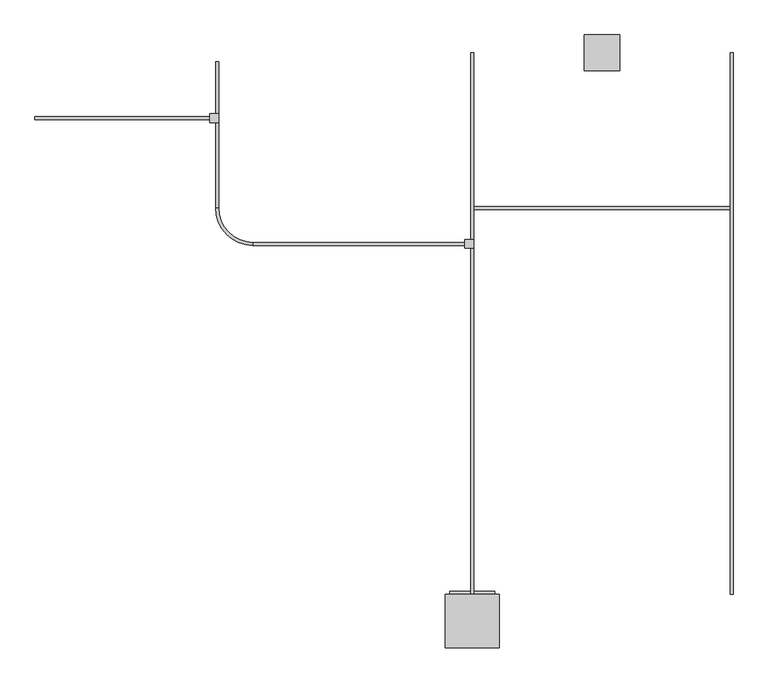
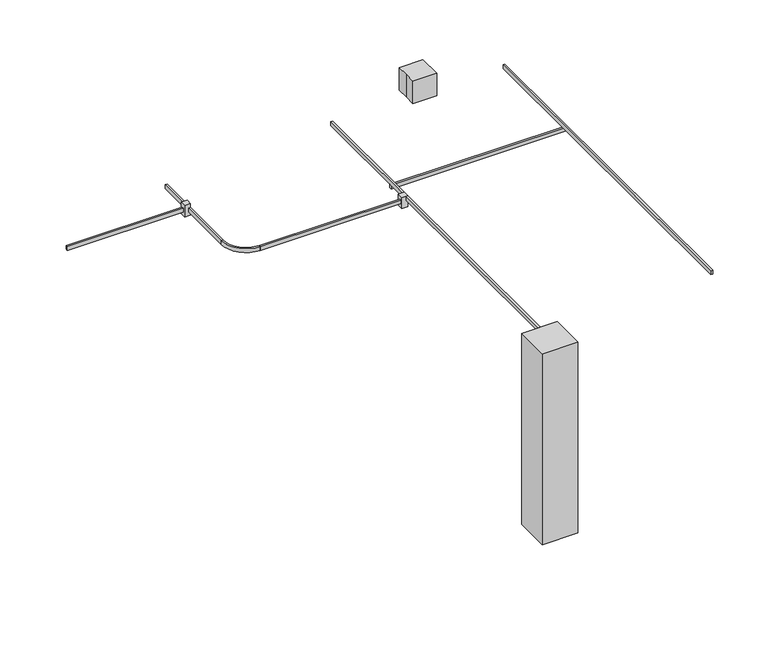
"""IFC4 building model written with IfcOpenShell, lengths in millimetres: proxy geometry, A1205 - Lift System, Overhead, Patient Room w-Bath-mirror : A1205 - Lift System, Overhead, Patient Room w-Bath-mirror."""

from ifc_helpers import new_model, si_unit, point, frame, frame_2d, origin, origin_with_axes, place, context, project, spatial, polyline, circle_curve, trimmed, segment, composite_curve, outline, extrude, source, transform, mapped, element, save


def specialty_equipment_7046e059(model_context):
    return source(origin(), model_context, "Body", "SweptSolid", [
        extrude(outline(polyline([(-3338.4200386, -545.1376019), (-3338.4200386, -570.5376019), (-4825.7229408, -570.5376019), (-4825.7229408, -545.1376019), (-3338.4200386, -545.1376019)])), frame((0.0, 0.0, -101.6), z_axis=(0.0, 0.0, 1.0), x_axis=(1.0, 0.0, 0.0)), (0.0, 0.0, 1.0), 50.8),
        extrude(outline(polyline([(-3338.4200386, -519.7376019), (-3262.2200386, -519.7376019), (-3262.2200386, -595.9376019), (-3338.4200386, -595.9376019), (-3338.4200386, -519.7376019)])), frame((0.0, 0.0, -152.4), z_axis=(0.0, 0.0, 1.0), x_axis=(1.0, 0.0, 0.0)), (0.0, 0.0, 1.0), 152.4),
        extrude(outline(composite_curve([segment(trimmed(circle_curve(frame_2d((-2970.1200386, -1322.4686515)), 292.1), [point((-3262.2200386, -1322.4686515))], [point((-2970.1200386, -1614.5686515))], True, "CARTESIAN"), True, "CONTINUOUS"), segment(polyline([(-2970.1200386, -1614.5686515), (-2970.1200386, -1639.9686515)]), True, "CONTINUOUS"), segment(trimmed(circle_curve(frame_2d((-2970.1200386, -1322.4686515)), 317.5), [point((-2970.1200386, -1639.9686515))], [point((-3287.6200386, -1322.4686515))], False, "CARTESIAN"), True, "CONTINUOUS"), segment(polyline([(-3287.6200386, -1322.4686515), (-3262.2200386, -1322.4686515)]), True, "CONTINUOUS")], self_intersect=False)), frame((0.0, 0.0, -101.6), z_axis=(0.0, 0.0, 1.0), x_axis=(1.0, 0.0, 0.0)), (0.0, 0.0, 1.0), 50.8),
        extrude(outline(polyline([(-3262.2200386, -1322.4686515), (-3287.6200386, -1322.4686515), (-3287.6200386, -75.2376019), (-3262.2200386, -75.2376019), (-3262.2200386, -1322.4686515)])), frame((0.0, 0.0, -101.6), z_axis=(0.0, 0.0, 1.0), x_axis=(1.0, 0.0, 0.0)), (0.0, 0.0, 1.0), 50.8),
        extrude(outline(polyline([(-1294.2912788, -4585.4992972), (-913.2912788, -4585.4992972), (-913.2912788, -4610.8992972), (-1294.2912788, -4610.8992972), (-1294.2912788, -4585.4992972)])), frame((0.0, 0.0, -2511.7688632), z_axis=(0.0, 0.0, 1.0), x_axis=(1.0, 0.0, 0.0)), (0.0, 0.0, 1.0), 2410.1688632),
        extrude(outline(polyline([(-875.1912788, -5068.0992972), (-1332.3912788, -5068.0992972), (-1332.3912788, -4610.8992972), (-875.1912788, -4610.8992972), (-875.1912788, -5068.0992972)])), frame((0.0, 0.0, -2590.8), z_axis=(0.0, 0.0, 1.0), x_axis=(1.0, 0.0, 0.0)), (0.0, 0.0, 1.0), 2590.8),
        extrude(outline(polyline([(-1167.2912788, -1589.1686515), (-1091.0912788, -1589.1686515), (-1091.0912788, -1665.3686515), (-1167.2912788, -1665.3686515), (-1167.2912788, -1589.1686515)])), frame((0.0, 0.0, -152.4), z_axis=(0.0, 0.0, 1.0), x_axis=(1.0, 0.0, 0.0)), (0.0, 0.0, 1.0), 152.4),
        extrude(outline(polyline([(-2970.1200386, -1639.9686515), (-2970.1200386, -1614.5686515), (-1167.2912788, -1614.5686515), (-1167.2912788, -1639.9686515), (-2970.1200386, -1639.9686515)])), frame((0.0, 0.0, -101.6), z_axis=(0.0, 0.0, 1.0), x_axis=(1.0, 0.0, 0.0)), (0.0, 0.0, 1.0), 50.8),
        extrude(outline(polyline([(-1091.0912788, -4610.8992972), (-1116.4912788, -4610.8992972), (-1116.4912788, 0.0), (-1091.0912788, 0.0), (-1091.0912788, -4610.8992972)])), frame((0.0, 0.0, -50.8), z_axis=(0.0, 0.0, 1.0), x_axis=(1.0, 0.0, 0.0)), (0.0, 0.0, 1.0), 50.8),
        extrude(outline(polyline([(1116.4912788, -1309.7686515), (1116.4912788, -1335.1686515), (-1116.4912788, -1335.1686515), (-1116.4912788, -1309.7686515), (1116.4912788, -1309.7686515)])), frame((0.0, 0.0, -101.6), z_axis=(0.0, 0.0, 1.0), x_axis=(1.0, 0.0, 0.0)), (0.0, 0.0, 1.0), 50.8),
        extrude(outline(polyline([(1116.4912788, -4610.8992972), (1091.0912788, -4610.8992972), (1091.0912788, 0.0), (1116.4912788, 0.0), (1116.4912788, -4610.8992972)])), frame((0.0, 0.0, -50.8), z_axis=(0.0, 0.0, 1.0), x_axis=(1.0, 0.0, 0.0)), (0.0, 0.0, 1.0), 50.8),
        extrude(outline(polyline([(-152.4, 152.4), (152.4, 152.4), (152.4, -152.4), (-152.4, -152.4), (-152.4, 0.0), (-152.4, 152.4)])), origin_with_axes(), (0.0, 0.0, 1.0), 304.8),
    ])


if __name__ == "__main__":
    model = new_model("IFC4")
    model_context = context("Model", 3, world=origin())
    ifc_project = project(units=[si_unit("LENGTHUNIT", "METRE", prefix="MILLI")], contexts=[model_context])
    site = spatial("IfcSite", under=ifc_project)
    building = spatial("IfcBuilding", under=site)
    placement = place(None, origin())
    specialty_equipment_shape = specialty_equipment_7046e059(model_context)
    element("IfcBuildingElementProxy", 1, Name="A1205 - Lift System, Overhead, Patient Room w-Bath-mirror : A1205 - Lift System, Overhead, Patient Room w-Bath-mirror", ObjectType="A1205 - Lift System, Overhead, Patient Room w-Bath-mirror : A1205 - Lift System, Overhead, Patient Room w-Bath-mirror", at=placement, inside=building, context=model_context, shape_type="MappedRepresentation", body=[
        mapped(specialty_equipment_shape, transform((0.0, 0.0, 0.0), x_axis=(1.0, 0.0, 0.0), y_axis=(0.0, 1.0, 0.0), z_axis=(0.0, 0.0, 1.0))),
    ])
    save(model, "model.ifc")

# Revit data of these elements
# Type "A1205 - Lift System, Overhead, Patient Room w-Bath-mirror : A1205 - Lift System, Overhead, Patient Room w-Bath-mirror"
#   Watts2 = "0"
#   Watts1 = "600"
#   Unit_Issue = "EA"
#   UTIL_6_Misc = "J"
#   UTIL_5_NonMedGas = "-"
#   UTIL_4_MiscGas = "-"
#   UTIL_3_MedGas = "-"
#   UTIL_2_Elec = "F"
#   UTIL_1_WaterDrain = "-"
#   Nomenclature = "Lift System, Overhead, Patient Room w/Bath"
#   NSN = ""
#   Location [instance default] = ""
#   JSN = "A1205"
#   Fund_Source_VA = "-"
#   Fund_Source_Navy = "-"
#   Fund_Source_Army = "-"
#   Fund_Source_AF = "-"
#   ELEC_Volts2 = "0"
#   ELEC_Volts1 = "120"
#   ELEC_Phase2 = "0"
#   ELEC_Phase1 = "1"
#   ELEC_HertzSwitch = "-1"
#   ELEC_HertzDependent = "0"
#   ELEC_Hertz = "0"
#   ELEC_Amps2 = "0"
#   ELEC_Amps1 = "5"
#   DetailDescription = "An overhead rail system specifically designed for patient lifting and movement for a single bed patient room including the bathroom. The system will consist of recessed or ceiling mounted primary and secondary rails, lift motor with rolling carriage, patient harness or seat, and a hand controller or control box with charger. System will facilitate lifting and movement of patient to and from bed to gurney, chair, bath, commode, or other requirement. Minimum lift capability is 550 pounds. Custom design of track layout by manufacturer is essential to meet individual facility requirements."
#   CAT_VA = "A"
#   CAT_Navy = "A"
#   CAT_IHS = "-"
#   CAT_Army = "A"
#   CAT_AF = "A"
#   BTUperhour = "0"
#   Weight_IP = 0
#   DIM_Width_IP = 1' - 0"
#   DIM_Height_IP = 1' - 0"
#   DIM_Depth_IP = 1' - 0"
#   CustonLength3 [instance default] = 5' - 3"
#   CustomLength4 [instance default] = 5' - 0"
#   CustomLength2 [instance default] = 6' - 3 1/2"
#   CustomLength [instance default] = 6' - 5"
#   CustomDepth3 [instance default] = 3' - 0"
#   CustomDepth2 [instance default] = 9' - 0"
#   CustomDepth [instance default] = 9' - 0 1/2"
# Element 1 (IfcBuildingElementProxy, "A1205 - Lift System, Overhead, Patient Room w-Bath-mirror : A1205 - Lift System, Overhead, Patient Room w-Bath-mirror")
#   Location = "BRMS1"
#   CustonLength3 = 5' - 1.55523"
#   CustomLength4 = 7' - 1.9127"
#   CustomLength2 = 6' - 1.97751"
#   CustomLength = 5' - 10.27979"
#   CustomDepth3 = 5' - 3.56569"
#   CustomDepth2 = 15' - 1.53147"
#   CustomDepth = 4' - 1.10358"
#   Materials on its faces: "EquipSpace"
# Materials
#   "EquipSpace": class "Unassigned", colour RGB 221 217 195, transparency 0.5
